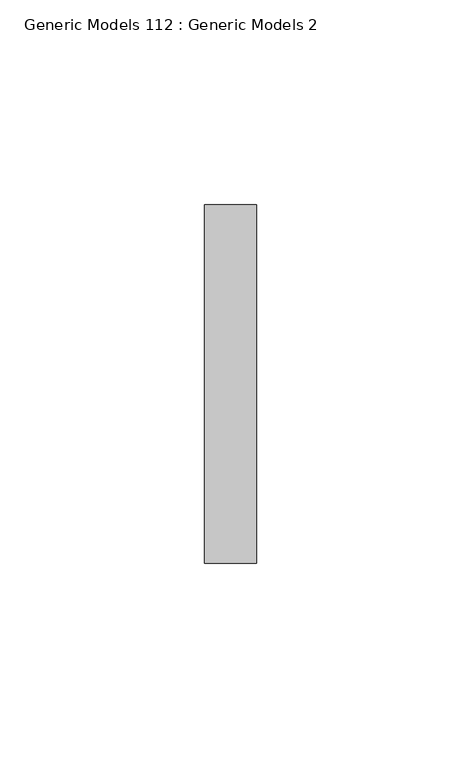
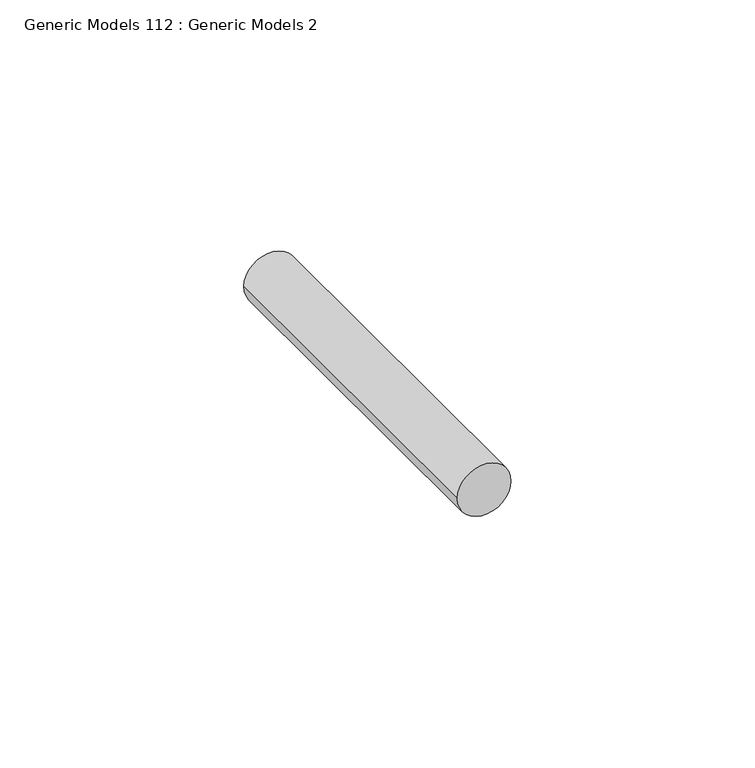
"""IFC4 building model written with IfcOpenShell, lengths in millimetres: proxy geometry, Generic Models 112 : Generic Models 2."""

from ifc_helpers import new_model, si_unit, point, frame, frame_2d, origin, place, context, project, spatial, circle_curve, trimmed, segment, composite_curve, outline, extrude, source, transform, mapped, element, save


def generic_models_112_generic_models_2_10aca697(model_context):
    return source(origin(), model_context, "Body", "SweptSolid", [
        extrude(outline(composite_curve([segment(trimmed(circle_curve(frame_2d((37688.9033735, 6459.3346014)), 6.35), [point((37688.9033735, 6465.6846014))], [point((37688.9033735, 6452.9846014))], False, "CARTESIAN"), True, "CONTINUOUS"), segment(trimmed(circle_curve(frame_2d((37688.9033735, 6459.3346014)), 6.35), [point((37688.9033735, 6452.9846014))], [point((37688.9033735, 6465.6846014))], False, "CARTESIAN"), True, "CONTINUOUS")], self_intersect=False)), frame((0.0, 1848.3666731, 0.0), z_axis=(0.0, 1.0, 0.0), x_axis=(0.0, 0.0, 1.0)), (0.0, 0.0, 1.0), 87.551022),
    ])


if __name__ == "__main__":
    model = new_model("IFC4")
    model_context = context("Model", 3, world=origin())
    ifc_project = project(units=[si_unit("LENGTHUNIT", "METRE", prefix="MILLI")], contexts=[model_context])
    site = spatial("IfcSite", under=ifc_project)
    building = spatial("IfcBuilding", under=site)
    placement = place(None, origin())
    generic_models_112_generic_models_2_shape = generic_models_112_generic_models_2_10aca697(model_context)
    element("IfcBuildingElementProxy", 1, Name="Generic Models 112 : Generic Models 2", ObjectType="Generic Models 112 : Generic Models 2", at=placement, inside=building, context=model_context, shape_type="MappedRepresentation", body=[
        mapped(generic_models_112_generic_models_2_shape, transform((0.0, 0.0, 0.0), x_axis=(1.0, 0.0, 0.0), y_axis=(0.0, 1.0, 0.0), z_axis=(0.0, 0.0, 1.0))),
    ])
    save(model, "model.ifc")

# Revit data of these elements
# Element 1 (IfcBuildingElementProxy, "Generic Models 112 : Generic Models 2")
#   Materials on its faces: "S.S. LAG BOLT - SEE STRUCT. DWGS"
# Materials
#   "S.S. LAG BOLT - SEE STRUCT. DWGS": class "Generic", colour RGB 120 120 120, transparency 0, Cost = 0
